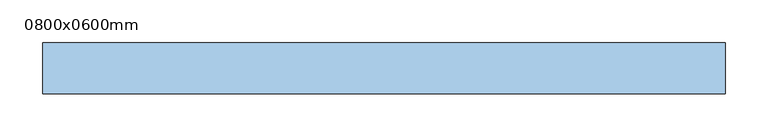
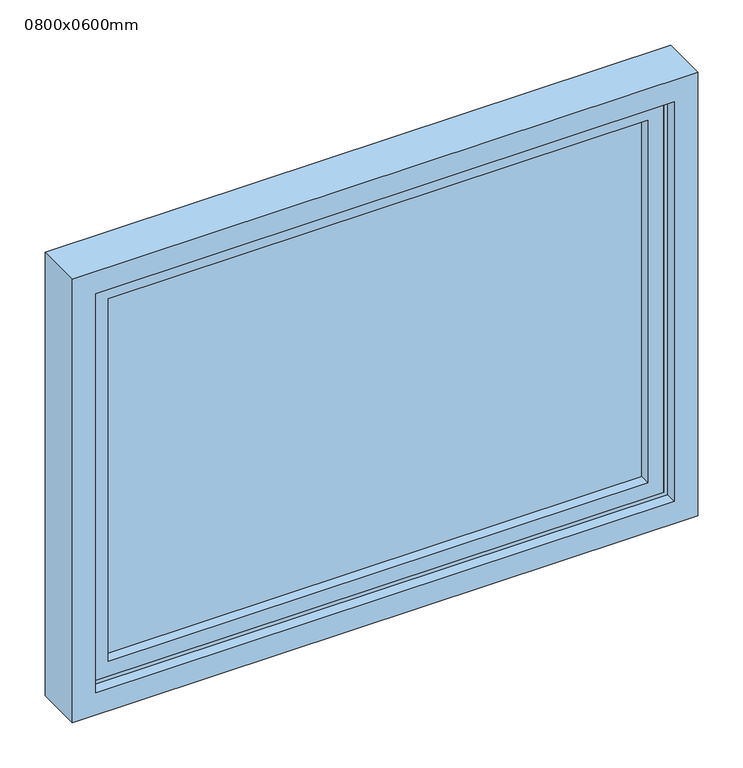
"""IFC4 building model written with IfcOpenShell, lengths in millimetres: window geometry, Janela Maxim-air - 1 Módulo : 0800x0600mm."""

from ifc_helpers import new_model, si_unit, frame, origin, place, context, project, spatial, polyline, outline, extrude, faceted_brep, source, transform, mapped, element, save


def window_0800x0600mm_eab3bed5(model_context):
    return source(origin(), model_context, "Body", "SolidModel", [
        extrude(outline(polyline([(-352.0, -24.120858), (352.0, -24.120858), (352.0, -31.120858), (-352.0, -31.120858), (-352.0, -24.120858)])), frame((0.0, 0.0, 1048.0), z_axis=(0.0, 0.0, 1.0), x_axis=(1.0, 0.0, 0.0)), (0.0, 0.0, 1.0), 504.0),
        faceted_brep([(345.0, -45.120858, 1545.0), (345.0, -31.120858, 1545.0), (345.0, -31.120858, 1055.0), (345.0, -45.120858, 1055.0), (352.0, -31.120858, 1552.0), (352.0, -24.120858, 1552.0), (352.0, -24.120858, 1048.0), (352.0, -31.120858, 1048.0), (345.0, -24.120858, 1545.0), (345.0, -10.120858, 1545.0), (345.0, -10.120858, 1055.0), (345.0, -24.120858, 1055.0), (365.0, -10.120858, 1565.0), (365.0, -45.120858, 1565.0), (365.0, -45.120858, 1035.0), (365.0, -10.120858, 1035.0), (-345.0, -31.120858, 1055.0), (-345.0, -45.120858, 1055.0), (-352.0, -24.120858, 1048.0), (-352.0, -31.120858, 1048.0), (-345.0, -10.120858, 1055.0), (-345.0, -24.120858, 1055.0), (-365.0, -45.120858, 1035.0), (-365.0, -10.120858, 1035.0), (-345.0, -31.120858, 1545.0), (-345.0, -45.120858, 1545.0), (-352.0, -24.120858, 1552.0), (-352.0, -31.120858, 1552.0), (-345.0, -10.120858, 1545.0), (-345.0, -24.120858, 1545.0), (-365.0, -45.120858, 1565.0), (-365.0, -10.120858, 1565.0)], [[[0, 1, 2, 3]], [[4, 5, 6, 7]], [[8, 9, 10, 11]], [[12, 13, 14, 15]], [[3, 2, 16, 17]], [[7, 6, 18, 19]], [[11, 10, 20, 21]], [[15, 14, 22, 23]], [[17, 16, 24, 25]], [[19, 18, 26, 27]], [[21, 20, 28, 29]], [[23, 22, 30, 31]], [[13, 30, 22, 14], [3, 17, 25, 0]], [[25, 24, 1, 0]], [[7, 19, 27, 4], [1, 24, 16, 2]], [[27, 26, 5, 4]], [[5, 26, 18, 6], [11, 21, 29, 8]], [[29, 28, 9, 8]], [[15, 23, 31, 12], [9, 28, 20, 10]], [[31, 30, 13, 12]]]),
        faceted_brep([(365.0, -45.120858, 1565.0), (365.0, -10.120858, 1565.0), (365.0, -10.120858, 1035.0), (365.0, -45.120858, 1035.0), (360.0, -10.120858, 1560.0), (360.0, -5.120858, 1560.0), (360.0, -5.120858, 1040.0), (360.0, -10.120858, 1040.0), (370.0, -5.120858, 1570.0), (370.0, -45.120858, 1570.0), (370.0, -45.120858, 1030.0), (370.0, -5.120858, 1030.0), (-365.0, -10.120858, 1035.0), (-365.0, -45.120858, 1035.0), (-360.0, -5.120858, 1040.0), (-360.0, -10.120858, 1040.0), (-370.0, -45.120858, 1030.0), (-370.0, -5.120858, 1030.0), (-365.0, -10.120858, 1565.0), (-365.0, -45.120858, 1565.0), (-360.0, -5.120858, 1560.0), (-360.0, -10.120858, 1560.0), (-370.0, -45.120858, 1570.0), (-370.0, -5.120858, 1570.0)], [[[0, 1, 2, 3]], [[4, 5, 6, 7]], [[8, 9, 10, 11]], [[3, 2, 12, 13]], [[7, 6, 14, 15]], [[11, 10, 16, 17]], [[13, 12, 18, 19]], [[15, 14, 20, 21]], [[17, 16, 22, 23]], [[9, 22, 16, 10], [3, 13, 19, 0]], [[19, 18, 1, 0]], [[1, 18, 12, 2], [7, 15, 21, 4]], [[21, 20, 5, 4]], [[11, 17, 23, 8], [5, 20, 14, 6]], [[23, 22, 9, 8]]]),
        faceted_brep([(400.0, -0.120858, 1600.0), (400.0, -60.120858, 1600.0), (400.0, -60.120858, 1000.0), (400.0, -0.120858, 1000.0), (-400.0, -60.120858, 1600.0), (-400.0, -60.120858, 1000.0), (370.0, -60.120858, 1030.0), (-370.0, -60.120858, 1030.0), (-370.0, -60.120858, 1570.0), (370.0, -60.120858, 1570.0), (-400.0, -0.120858, 1000.0), (-400.0, -0.120858, 1600.0), (360.0, -0.120858, 1560.0), (-360.0, -0.120858, 1560.0), (-360.0, -0.120858, 1040.0), (360.0, -0.120858, 1040.0), (370.0, -5.120858, 1570.0), (370.0, -5.120858, 1030.0), (-370.0, -5.120858, 1570.0), (-370.0, -5.120858, 1030.0), (360.0, -5.120858, 1040.0), (-360.0, -5.120858, 1040.0), (-360.0, -5.120858, 1560.0), (360.0, -5.120858, 1560.0)], [[[0, 1, 2, 3]], [[1, 4, 5, 2], [6, 7, 8, 9]], [[3, 2, 5, 10]], [[3, 10, 11, 0], [12, 13, 14, 15]], [[9, 16, 17, 6]], [[16, 18, 19, 17], [20, 21, 22, 23]], [[6, 17, 19, 7]], [[10, 5, 4, 11]], [[7, 19, 18, 8]], [[23, 12, 15, 20]], [[20, 15, 14, 21]], [[21, 14, 13, 22]], [[11, 4, 1, 0]], [[8, 18, 16, 9]], [[22, 13, 12, 23]]]),
    ])


if __name__ == "__main__":
    model = new_model("IFC4")
    model_context = context("Model", 3, world=origin())
    ifc_project = project(units=[si_unit("LENGTHUNIT", "METRE", prefix="MILLI")], contexts=[model_context])
    site = spatial("IfcSite", under=ifc_project)
    building = spatial("IfcBuilding", under=site)
    placement = place(None, origin())
    window_0800x0600mm_shape = window_0800x0600mm_eab3bed5(model_context)
    element("IfcWindow", 1, ObjectType="Janela Maxim-air - 1 Módulo : 0800x0600mm", at=placement, inside=building, context=model_context, shape_type="MappedRepresentation", body=[
        mapped(window_0800x0600mm_shape, transform((0.0, 0.0, 0.0), x_axis=(1.0, 0.0, 0.0), y_axis=(0.0, 1.0, 0.0), z_axis=(0.0, 0.0, 1.0))),
    ])
    save(model, "model.ifc")

# Revit data of these elements
# Type "Janela Maxim-air - 1 Módulo : 0800x0600mm"
#   Type Mark = ""
#   SINAPI = ""
#   Módulo Básico M = 10.00 cm
#   Largura de Coordenação Modular CM = 80.00 cm
#   Largura Painel = 74.00 cm
#   Largura Batente = 6.00 cm
#   Altura de Coordenação Modular CM = 60.00 cm
#   Altura Peitoril = 100.00 cm
#   Altura Painel = 54.00 cm
#   Height = 60.00 cm
#   Width = 80.00 cm
#   Número de Módulos Básicos nM Largura = 8
#   Número de Módulos Básico nM Altura = 6
#   Material Quadro = Metal - Alumínio
#   Material Painel = Vidro
#   Wall Closure = (empty or 0)
#   Assembly Code = ""
# Element 1 (IfcWindow, "Janela Maxim-air - 1 Módulo : 0800x0600mm")
#   Materials on its faces: "Metal - Alumínio", "Vidro"
# Materials
#   "Metal - Alumínio": class "Metal", colour RGB 244 244 244, transparency 0
#   "Vidro": class "Vidro", colour RGB 230 230 230, transparency 0.75, Cost = 0
